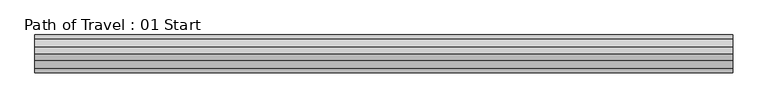
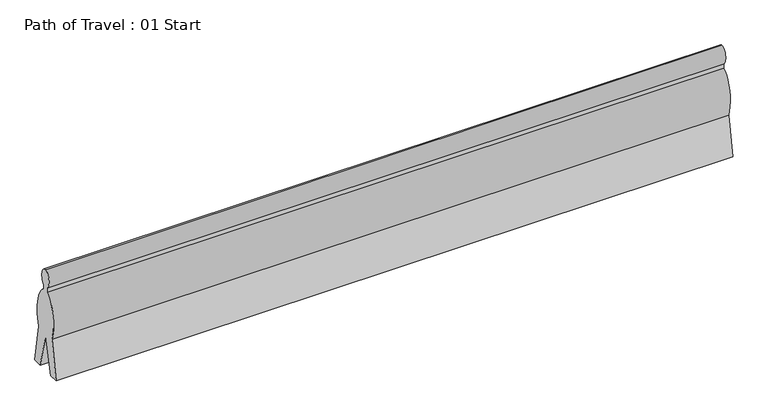
"""IFC4 building model written with IfcOpenShell, lengths in millimetres: proxy geometry, Path of Travel : 01 Start."""

import ifcopenshell
import ifcopenshell.guid

model = None  # the IFC model being written
_history = None  # IfcOwnerHistory: only IFC2X3 demands one
_inside = {}  # id of a spatial element -> (the spatial element, [elements in it])
_under = {}  # id of a project, library or spatial element -> (it, [spatial elements below it])
_declared = {}  # id of a project -> (the project, [libraries it declares])
_typed = {}  # id of a type object -> (the type object, [elements of that type])
_made_of = {}  # id of a material, layer set ... -> (it, [elements and type objects made of it])


def new_model(schema):
    """Start an empty IFC model of exactly this schema.

    Asked for "IFC4X3", IfcOpenShell would pick the latest addendum, in which some entities
    have other attributes; the version numbers below select the first issue.
    IFC2X3 requires an IfcOwnerHistory on every rooted entity: one is made here for all.
    """
    global model, _history
    if schema == "IFC4X3":
        model = ifcopenshell.file(schema_version=(4, 3, 0, 0))
    else:
        model = ifcopenshell.file(schema=schema)
    _inside.clear()
    _under.clear()
    _declared.clear()
    _typed.clear()
    _made_of.clear()
    _history = None
    if model.schema == "IFC2X3":
        org = make("IfcOrganization", Name="unknown")
        user = make(
            "IfcPersonAndOrganization",
            ThePerson=make("IfcPerson", FamilyName="unknown"),
            TheOrganization=org,
        )
        app = make(
            "IfcApplication",
            ApplicationDeveloper=org,
            Version="unknown",
            ApplicationFullName="unknown",
            ApplicationIdentifier="unknown",
        )
        _history = make(
            "IfcOwnerHistory",
            OwningUser=user,
            OwningApplication=app,
            ChangeAction="ADDED",
            CreationDate=0,
        )
    return model


def make(cls, **values):
    """One entity of the class cls with the attributes given. An attribute that is None is left unset."""
    return model.create_entity(
        cls, **{name: value for name, value in values.items() if value is not None}
    )


def rooted(cls, **values):
    """An entity with a GlobalId (a new one), such as an element, a storey or a relation."""
    return make(cls, GlobalId=ifcopenshell.guid.new(), OwnerHistory=_history, **values)


def si_unit(unit_type, name, prefix=None):
    """IfcSIUnit, for example si_unit("LENGTHUNIT", "METRE", prefix="MILLI")."""
    return make("IfcSIUnit", UnitType=unit_type, Prefix=prefix, Name=name)


def assignment(units):
    """IfcUnitAssignment: the units of a project."""
    return None if units is None else make("IfcUnitAssignment", Units=units)


def point(xyz):
    """IfcCartesianPoint."""
    return None if xyz is None else make("IfcCartesianPoint", Coordinates=xyz)


def direction(xyz):
    """IfcDirection."""
    return None if xyz is None else make("IfcDirection", DirectionRatios=xyz)


def frame(location, z_axis=None, x_axis=None):
    """IfcAxis2Placement3D, a coordinate frame: its origin and axes. An axis left out is left unset."""
    return make(
        "IfcAxis2Placement3D",
        Location=point(location),
        Axis=direction(z_axis),
        RefDirection=direction(x_axis),
    )


def origin():
    """The frame at (0, 0, 0) with its axes left unset."""
    return frame((0.0, 0.0, 0.0))


def place(relative_to, where):
    """IfcLocalPlacement: puts the frame where relative to a parent placement (None: the world)."""
    return make(
        "IfcLocalPlacement", PlacementRelTo=relative_to, RelativePlacement=where
    )


def context(
    kind, dimensions, precision=None, world=None, true_north=None, identifier=None
):
    """IfcGeometricRepresentationContext, for example the 3D "Model" context."""
    return make(
        "IfcGeometricRepresentationContext",
        ContextIdentifier=identifier,
        ContextType=kind,
        CoordinateSpaceDimension=dimensions,
        Precision=precision,
        WorldCoordinateSystem=world,
        TrueNorth=true_north,
    )


def project(units=None, contexts=None):
    """IfcProject with its units and contexts."""
    return rooted(
        "IfcProject",
        Name="project",
        RepresentationContexts=contexts,
        UnitsInContext=assignment(units),
    )


def spatial(cls, under=None, at=None, **own):
    """A site, building, storey or space (cls), placed at a placement, below another one or the project."""
    s = rooted(cls, ObjectPlacement=at, **own)
    if under is not None:
        _under.setdefault(under.id(), (under, []))[1].append(s)
    return s


def ellipse_curve(where, semi_axis1, semi_axis2):
    """IfcEllipse in the frame where."""
    return make(
        "IfcEllipse", Position=where, SemiAxis1=semi_axis1, SemiAxis2=semi_axis2
    )


def trimmed(basis, trim1, trim2, sense, master):
    """IfcTrimmedCurve: the piece of a basis curve between two trims."""
    return make(
        "IfcTrimmedCurve",
        BasisCurve=basis,
        Trim1=trim1,
        Trim2=trim2,
        SenseAgreement=sense,
        MasterRepresentation=master,
    )


def shape(context_of_items, identifier, shape_type, items):
    """IfcShapeRepresentation: the items that make up one representation, for example the "Body"."""
    return make(
        "IfcShapeRepresentation",
        ContextOfItems=context_of_items,
        RepresentationIdentifier=identifier,
        RepresentationType=shape_type,
        Items=items,
    )


def source(mapping_origin, context_of_items, identifier, shape_type, items):
    """IfcRepresentationMap: a shape defined once, which mapped items show again and again."""
    return make(
        "IfcRepresentationMap",
        MappingOrigin=mapping_origin,
        MappedRepresentation=shape(context_of_items, identifier, shape_type, items),
    )


def transform(
    local_origin,
    x_axis=None,
    y_axis=None,
    z_axis=None,
    scale=None,
    scale2=None,
    scale3=None,
    uniform=True,
):
    """IfcCartesianTransformationOperator3D, or its non-uniform kind. x_axis, y_axis, z_axis: its Axis1, 2, 3."""
    if uniform:
        return make(
            "IfcCartesianTransformationOperator3D",
            Axis1=direction(x_axis),
            Axis2=direction(y_axis),
            LocalOrigin=point(local_origin),
            Scale=scale,
            Axis3=direction(z_axis),
        )
    return make(
        "IfcCartesianTransformationOperator3DnonUniform",
        Axis1=direction(x_axis),
        Axis2=direction(y_axis),
        LocalOrigin=point(local_origin),
        Scale=scale,
        Axis3=direction(z_axis),
        Scale2=scale2,
        Scale3=scale3,
    )


def mapped(mapping_source, mapping_target):
    """IfcMappedItem: shows the shape of a source again, moved by a transform."""
    return make(
        "IfcMappedItem", MappingSource=mapping_source, MappingTarget=mapping_target
    )


def made_of(thing, what):
    """Note that an element or type object is made of a material, layer set ...; save() writes the relation."""
    if what is not None:
        _made_of.setdefault(what.id(), (what, []))[1].append(thing)
    return thing


def element(
    cls,
    number,
    at=None,
    inside=None,
    cuts=None,
    type_object=None,
    material=None,
    context=None,
    identifier="Body",
    shape_type=None,
    held_by="IfcProductDefinitionShape",
    body=None,
    shapes=None,
    **own,
):
    """One element of the class cls, such as IfcWall. Its Tag is "e" and its number.

    at: its placement. inside: the storey or other place that contains it. cuts: it is an
    opening in that element (IfcRelVoidsElement). A single representation is given by context,
    identifier, shape_type and body (its items); several are given by shapes. held_by: the class
    of the entity that holds the representations. save() writes the other relations.
    """
    e = rooted(cls, Tag="e%d" % number, ObjectPlacement=at, **own)
    if body is not None:
        shapes = [shape(context, identifier, shape_type, body)]
    if shapes is not None:
        e.Representation = make(held_by, Representations=shapes)
    if inside is not None:
        _inside.setdefault(inside.id(), (inside, []))[1].append(e)
    if cuts is not None:
        rooted(
            "IfcRelVoidsElement", RelatingBuildingElement=cuts, RelatedOpeningElement=e
        )
    if type_object is not None:
        _typed.setdefault(type_object.id(), (type_object, []))[1].append(e)
    return made_of(e, material)


def aggregate(whole, parts):
    """IfcRelAggregates: a whole, such as a stair, and the parts it consists of."""
    return rooted("IfcRelAggregates", RelatingObject=whole, RelatedObjects=parts)


def save(model, path):
    """Write the relations noted so far, then the file.

    IfcRelAggregates (storeys below a building ...), IfcRelContainedInSpatialStructure (elements
    in a storey), IfcRelDefinesByType, IfcRelAssociatesMaterial and IfcRelDeclares: one each for
    every whole, place, type object, material and project.
    """
    for whole, parts in _under.values():
        aggregate(whole, parts)
    for where, things in _inside.values():
        rooted(
            "IfcRelContainedInSpatialStructure",
            RelatedElements=things,
            RelatingStructure=where,
        )
    for kind, things in _typed.values():
        rooted("IfcRelDefinesByType", RelatedObjects=things, RelatingType=kind)
    for what, things in _made_of.values():
        rooted("IfcRelAssociatesMaterial", RelatedObjects=things, RelatingMaterial=what)
    for by, libraries in _declared.values():
        rooted("IfcRelDeclares", RelatingContext=by, RelatedDefinitions=libraries)
    model.write(path)


def plane_surface(at):
    """IfcPlane: the flat surface through the origin of the frame at, square to its z axis."""
    return make("IfcPlane", Position=at)


def extruded_surface(curve, direction_of_extrusion, depth):
    """IfcSurfaceOfLinearExtrusion: the curve pushed along a direction by depth."""
    return make(
        "IfcSurfaceOfLinearExtrusion",
        SweptCurve=make("IfcArbitraryOpenProfileDef", ProfileType="CURVE", Curve=curve),
        ExtrudedDirection=direction(direction_of_extrusion),
        Depth=depth,
    )


def advanced_brep(points, edges, surfaces, faces):
    """IfcAdvancedBrep: a solid bounded by faces that lie on surfaces and meet in shared edges.

    An edge is (start, end): straight between two places in points (the first is 0);
    or (start, end, curve); or (start, end, curve, False) where it runs against its curve.
    A face is (place in surfaces, loops), or (place, loops, False) where it looks against
    its surface's normal. A loop lists edges by number (the first is 1), with a minus sign
    where the edge is run from its end to its start. The first loop is the outer one.
    """
    corners = [point(p) for p in points]
    vertices = [make("IfcVertexPoint", VertexGeometry=c) for c in corners]
    made = []
    for start, end, *more in edges:
        made.append(
            make(
                "IfcEdgeCurve",
                EdgeStart=vertices[start],
                EdgeEnd=vertices[end],
                EdgeGeometry=more[0] if more else make("IfcPolyline", Points=[corners[start], corners[end]]),
                SameSense=more[1] if len(more) > 1 else True,
            )
        )
    hull = []
    for where, loops, *sense in faces:
        bounds = []
        for j, loop in enumerate(loops):
            ring = [make("IfcOrientedEdge", EdgeElement=made[abs(k) - 1], Orientation=k > 0) for k in loop]
            bounds.append(
                make(
                    "IfcFaceOuterBound" if j == 0 else "IfcFaceBound",
                    Bound=make("IfcEdgeLoop", EdgeList=ring),
                    Orientation=True,
                )
            )
        hull.append(make("IfcAdvancedFace", Bounds=bounds, FaceSurface=surfaces[where], SameSense=sense[0] if sense else True))
    return make("IfcAdvancedBrep", Outer=make("IfcClosedShell", CfsFaces=hull))


def path_of_travel_01_start_212660b2(model_context):
    return source(origin(), model_context, "Body", "AdvancedBrep", [
        advanced_brep(
        [(227.5554837, 0.0, 1727.2), (227.5554837, 42.9018657, 1436.6534209), (227.5554837, 42.9018657, 1363.4763406), (227.5554837, 184.1186263, 643.4144547), (227.5554837, 297.5699544, 0.0), (227.5554837, 145.6574193, 0.0), (227.5554837, 0.0, 584.2), (227.5554837, -145.6574193, 0.0), (227.5554837, -297.5699544, 0.0), (227.5554837, -184.1186263, 643.4144547), (227.5554837, -42.9018657, 1363.4763406), (227.5554837, -42.9018657, 1436.6534209), (11200.3554837, 0.0, 1727.2), (11200.3554837, -42.9018657, 1436.6534209), (11200.3554837, -42.9018657, 1363.4763406), (11200.3554837, -184.1186263, 643.4144547), (11200.3554837, -297.5699544, 0.0), (11200.3554837, -145.6574193, 0.0), (11200.3554837, 0.0, 584.2), (11200.3554837, 145.6574193, 0.0), (11200.3554837, 297.5699544, 0.0), (11200.3554837, 184.1186263, 643.4144547), (11200.3554837, 42.9018657, 1363.4763406), (11200.3554837, 42.9018657, 1436.6534209)],
        [
            (0, 1, ellipse_curve(frame((227.5554837, 0.0, 1574.8), z_axis=(-1.0, 0.0, 0.0), x_axis=(0.0, 0.0, 1.0)), 152.4, 101.6)),
            (1, 2),
            (2, 3, ellipse_curve(frame((227.5554837, 0.0, 914.4), z_axis=(-1.0, 0.0, 0.0), x_axis=(0.0, 0.0, -1.0)), 457.2, 228.6)),
            (3, 4),
            (4, 5),
            (5, 6),
            (6, 7),
            (7, 8),
            (8, 9),
            (9, 10, ellipse_curve(frame((227.5554837, 0.0, 914.4), z_axis=(-1.0, 0.0, 0.0), x_axis=(0.0, 0.0, -1.0)), 457.2, 228.6)),
            (10, 11),
            (11, 0, ellipse_curve(frame((227.5554837, 0.0, 1574.8), z_axis=(-1.0, 0.0, 0.0), x_axis=(0.0, 0.0, 1.0)), 152.4, 101.6)),
            (12, 13, ellipse_curve(frame((11200.3554837, 0.0, 1574.8), z_axis=(1.0, 0.0, 0.0), x_axis=(0.0, 0.0, 1.0)), 152.4, 101.6)),
            (13, 14),
            (14, 15, ellipse_curve(frame((11200.3554837, 0.0, 914.4), z_axis=(1.0, 0.0, 0.0), x_axis=(0.0, 0.0, -1.0)), 457.2, 228.6)),
            (15, 16),
            (16, 17),
            (17, 18),
            (18, 19),
            (19, 20),
            (20, 21),
            (21, 22, ellipse_curve(frame((11200.3554837, 0.0, 914.4), z_axis=(1.0, 0.0, 0.0), x_axis=(0.0, 0.0, -1.0)), 457.2, 228.6)),
            (22, 23),
            (23, 12, ellipse_curve(frame((11200.3554837, 0.0, 1574.8), z_axis=(1.0, 0.0, 0.0), x_axis=(0.0, 0.0, 1.0)), 152.4, 101.6)),
            (0, 12),
            (23, 1),
            (22, 2),
            (21, 3),
            (20, 4),
            (19, 5),
            (18, 6),
            (17, 7),
            (16, 8),
            (15, 9),
            (14, 10),
            (13, 11),
        ],
        [
            plane_surface(frame((227.5554837, 0.0, 0.0), z_axis=(-1.0, 0.0, 0.0), x_axis=(0.0, 0.0, 1.0))),
            plane_surface(frame((11200.3554837, 0.0, 0.0), z_axis=(1.0, 0.0, 0.0), x_axis=(0.0, 0.0, 1.0))),
            extruded_surface(trimmed(ellipse_curve(frame((11200.3554837, 0.0, 1574.8), z_axis=(-1.0, 0.0, 0.0), x_axis=(0.0, 0.0, 1.0)), 152.4, 101.6), [point((11200.3554837, 0.0, 1727.2))], [point((11200.3554837, 42.9018657, 1436.6534209))], True, "CARTESIAN"), (-10972.8, 0.0, 0.0), 10972.8),
            plane_surface(frame((227.5554837, 42.9018657, 1436.6534209), z_axis=(0.0, 1.0, 0.0), x_axis=(1.0, 0.0, 0.0))),
            extruded_surface(trimmed(ellipse_curve(frame((11200.3554837, 0.0, 914.4), z_axis=(-1.0, 0.0, 0.0), x_axis=(0.0, 0.0, -1.0)), 457.2, 228.6), [point((11200.3554837, 42.9018657, 1363.4763406))], [point((11200.3554837, 184.1186263, 643.4144547))], True, "CARTESIAN"), (-10972.8, 0.0, 0.0), 10972.8),
            plane_surface(frame((227.5554837, 184.1186263, 643.4144547), z_axis=(0.0, 0.9848077530122078, 0.17364817766693205), x_axis=(1.0, 0.0, 0.0))),
            plane_surface(frame((227.5554837, 297.5699544, 0.0), z_axis=(0.0, 0.0, -1.0), x_axis=(1.0, 0.0, 0.0))),
            plane_surface(frame((227.5554837, 145.6574193, 0.0), z_axis=(0.0, -0.9702957262760199, -0.2419218955995739), x_axis=(1.0, 0.0, 0.0))),
            plane_surface(frame((227.5554837, 0.0, 584.2), z_axis=(0.0, 0.9702957262759961, -0.24192189559966923), x_axis=(1.0, 0.0, 0.0))),
            plane_surface(frame((227.5554837, -145.6574193, 0.0), z_axis=(0.0, 0.0, -1.0), x_axis=(1.0, 0.0, 0.0))),
            plane_surface(frame((227.5554837, -297.5699544, 0.0), z_axis=(0.0, -0.984807753012208, 0.17364817766693066), x_axis=(1.0, 0.0, 0.0))),
            extruded_surface(trimmed(ellipse_curve(frame((11200.3554837, 0.0, 914.4), z_axis=(-1.0, 0.0, 0.0), x_axis=(0.0, 0.0, -1.0)), 457.2, 228.6), [point((11200.3554837, -184.1186263, 643.4144547))], [point((11200.3554837, -42.9018657, 1363.4763406))], True, "CARTESIAN"), (-10972.8, 0.0, 0.0), 10972.8),
            plane_surface(frame((227.5554837, -42.9018657, 1363.4763406), z_axis=(0.0, -1.0, 0.0), x_axis=(1.0, 0.0, 0.0))),
            extruded_surface(trimmed(ellipse_curve(frame((11200.3554837, 0.0, 1574.8), z_axis=(-1.0, 0.0, 0.0), x_axis=(0.0, 0.0, 1.0)), 152.4, 101.6), [point((11200.3554837, -42.9018657, 1436.6534209))], [point((11200.3554837, 0.0, 1727.2))], True, "CARTESIAN"), (-10972.8, 0.0, 0.0), 10972.8),
        ],
        [
            (0, [[1, 2, 3, 4, 5, 6, 7, 8, 9, 10, 11, 12]]),
            (1, [[13, 14, 15, 16, 17, 18, 19, 20, 21, 22, 23, 24]]),
            (2, [[-1, 25, -24, 26]]),
            (3, [[-2, -26, -23, 27]]),
            (4, [[-3, -27, -22, 28]]),
            (5, [[-4, -28, -21, 29]]),
            (6, [[-5, -29, -20, 30]]),
            (7, [[-6, -30, -19, 31]]),
            (8, [[-7, -31, -18, 32]]),
            (9, [[-8, -32, -17, 33]]),
            (10, [[-9, -33, -16, 34]]),
            (11, [[-10, -34, -15, 35]]),
            (12, [[-11, -35, -14, 36]]),
            (13, [[-12, -36, -13, -25]]),
        ],
    ),
    ])


if __name__ == "__main__":
    model = new_model("IFC4")
    model_context = context("Model", 3, world=origin())
    ifc_project = project(units=[si_unit("LENGTHUNIT", "METRE", prefix="MILLI")], contexts=[model_context])
    site = spatial("IfcSite", under=ifc_project)
    building = spatial("IfcBuilding", under=site)
    placement = place(None, origin())
    path_of_travel_01_start_shape = path_of_travel_01_start_212660b2(model_context)
    element("IfcBuildingElementProxy", 1, Name="Path of Travel : 01 Start", ObjectType="Path of Travel : 01 Start", at=placement, inside=building, context=model_context, shape_type="MappedRepresentation", body=[
        mapped(path_of_travel_01_start_shape, transform((0.0, 0.0, 0.0), x_axis=(1.0, 0.0, 0.0), y_axis=(0.0, 1.0, 0.0), z_axis=(0.0, 0.0, 1.0))),
    ])
    save(model, "model.ifc")

# Revit data of these elements
# Type "Path of Travel : 01 Start"
#   Path of Egress [instance default] = 4' - 0"
#   built-in parameter 1001306 [instance default] = 4 (stored number, unit not read)
#   Dot at Start = yes
#   Arrow in Middle = yes
#   Arrow at End = no
#   Egress Path = none
# Element 1 (IfcBuildingElementProxy, "Path of Travel : 01 Start")
#   Path of Egress = 36' - 0"
#   built-in parameter 1001306 = 36 (stored number, unit not read)
#   Materials on its faces: "Egress Path Solid"
# Materials
#   "Egress Path Solid": class "Unassigned", colour RGB 255 128 64, transparency 0.75, Comments = "Rendering appearance not upgraded "
